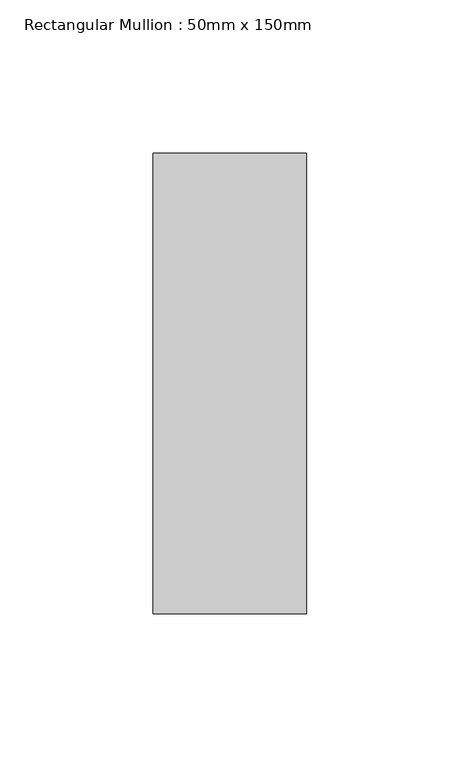
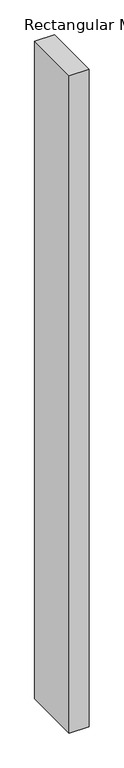
"""IFC4 building model written with IfcOpenShell, lengths in millimetres: member geometry, Rectangular Mullion : 50mm x 150mm."""

from ifc_helpers import new_model, si_unit, frame, origin, place, context, project, spatial, polyline, outline, extrude, source, transform, mapped, element, save


def rectangular_mullion_50mm_x_150mm_9a689882(model_context):
    return source(origin(), model_context, "Body", "SweptSolid", [
        extrude(outline(polyline([(25.0, 75.0), (25.0, -75.0), (-25.0, -75.0), (-25.0, 75.0), (25.0, 75.0)])), frame((0.0, 0.0, -1748.5454546), z_axis=(0.0, 0.0, 1.0), x_axis=(1.0, 0.0, 0.0)), (0.0, 0.0, 1.0), 1748.5454546),
    ])


if __name__ == "__main__":
    model = new_model("IFC4")
    model_context = context("Model", 3, world=origin())
    ifc_project = project(units=[si_unit("LENGTHUNIT", "METRE", prefix="MILLI")], contexts=[model_context])
    site = spatial("IfcSite", under=ifc_project)
    building = spatial("IfcBuilding", under=site)
    placement = place(None, origin())
    rectangular_mullion_50mm_x_150mm_shape = rectangular_mullion_50mm_x_150mm_9a689882(model_context)
    element("IfcMember", 1, ObjectType="Rectangular Mullion : 50mm x 150mm", at=placement, inside=building, context=model_context, shape_type="MappedRepresentation", body=[
        mapped(rectangular_mullion_50mm_x_150mm_shape, transform((0.0, 0.0, 0.0), x_axis=(1.0, 0.0, 0.0), y_axis=(0.0, 1.0, 0.0), z_axis=(0.0, 0.0, 1.0))),
    ])
    save(model, "model.ifc")

# Revit data of these elements
# Type "Rectangular Mullion : 50mm x 150mm"
#   built-in parameter 1007304 = 0.492126 (stored number, unit not read)
#   built-in parameter 1007301 = 0.082021 (stored number, unit not read)
#   built-in parameter 1007300 = 0.082021 (stored number, unit not read)
# Element 1 (IfcMember, "Rectangular Mullion : 50mm x 150mm")
#   Materials on its faces: "Aluminum"
# Materials
#   "Aluminum": class "Metal", colour RGB 244 244 244, transparency 0, Description = "Aluminum 6061", Cost = 0
